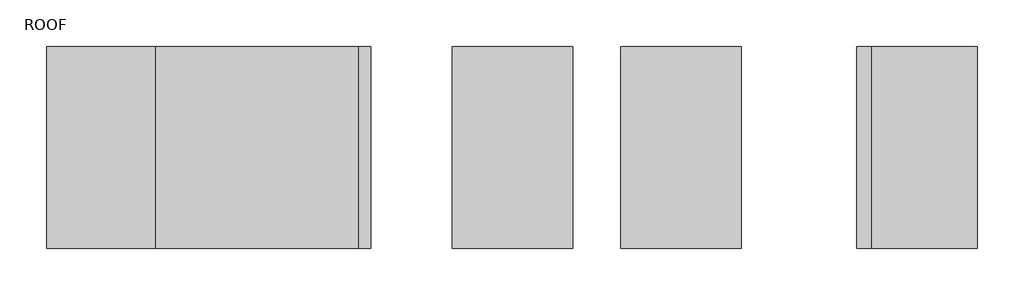
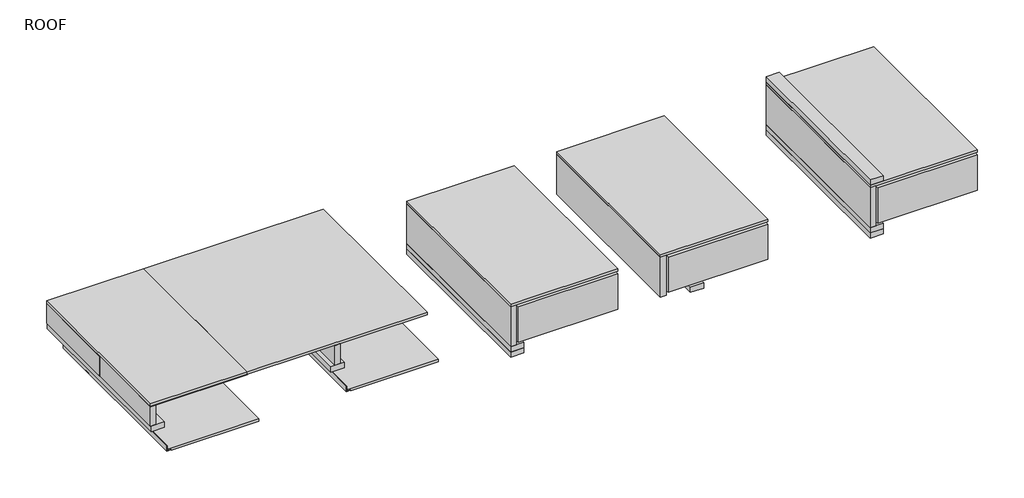
# One storey: 38 proxies.
"""IFC4 building model written with IfcOpenShell, lengths in millimetres."""

import ifcopenshell
import ifcopenshell.guid

model = None  # the IFC model being written
_history = None  # IfcOwnerHistory: only IFC2X3 demands one
_inside = {}  # id of a spatial element -> (the spatial element, [elements in it])
_under = {}  # id of a project, library or spatial element -> (it, [spatial elements below it])
_declared = {}  # id of a project -> (the project, [libraries it declares])
_typed = {}  # id of a type object -> (the type object, [elements of that type])
_made_of = {}  # id of a material, layer set ... -> (it, [elements and type objects made of it])


def new_model(schema):
    """Start an empty IFC model of exactly this schema.

    Asked for "IFC4X3", IfcOpenShell would pick the latest addendum, in which some entities
    have other attributes; the version numbers below select the first issue.
    IFC2X3 requires an IfcOwnerHistory on every rooted entity: one is made here for all.
    """
    global model, _history
    if schema == "IFC4X3":
        model = ifcopenshell.file(schema_version=(4, 3, 0, 0))
    else:
        model = ifcopenshell.file(schema=schema)
    _inside.clear()
    _under.clear()
    _declared.clear()
    _typed.clear()
    _made_of.clear()
    _history = None
    if model.schema == "IFC2X3":
        org = make("IfcOrganization", Name="unknown")
        user = make(
            "IfcPersonAndOrganization",
            ThePerson=make("IfcPerson", FamilyName="unknown"),
            TheOrganization=org,
        )
        app = make(
            "IfcApplication",
            ApplicationDeveloper=org,
            Version="unknown",
            ApplicationFullName="unknown",
            ApplicationIdentifier="unknown",
        )
        _history = make(
            "IfcOwnerHistory",
            OwningUser=user,
            OwningApplication=app,
            ChangeAction="ADDED",
            CreationDate=0,
        )
    return model


def make(cls, **values):
    """One entity of the class cls with the attributes given. An attribute that is None is left unset."""
    return model.create_entity(
        cls, **{name: value for name, value in values.items() if value is not None}
    )


def rooted(cls, **values):
    """An entity with a GlobalId (a new one), such as an element, a storey or a relation."""
    return make(cls, GlobalId=ifcopenshell.guid.new(), OwnerHistory=_history, **values)


def si_unit(unit_type, name, prefix=None):
    """IfcSIUnit, for example si_unit("LENGTHUNIT", "METRE", prefix="MILLI")."""
    return make("IfcSIUnit", UnitType=unit_type, Prefix=prefix, Name=name)


def assignment(units):
    """IfcUnitAssignment: the units of a project."""
    return None if units is None else make("IfcUnitAssignment", Units=units)


def point(xyz):
    """IfcCartesianPoint."""
    return None if xyz is None else make("IfcCartesianPoint", Coordinates=xyz)


def direction(xyz):
    """IfcDirection."""
    return None if xyz is None else make("IfcDirection", DirectionRatios=xyz)


def frame(location, z_axis=None, x_axis=None):
    """IfcAxis2Placement3D, a coordinate frame: its origin and axes. An axis left out is left unset."""
    return make(
        "IfcAxis2Placement3D",
        Location=point(location),
        Axis=direction(z_axis),
        RefDirection=direction(x_axis),
    )


def origin():
    """The frame at (0, 0, 0) with its axes left unset."""
    return frame((0.0, 0.0, 0.0))


def place(relative_to, where):
    """IfcLocalPlacement: puts the frame where relative to a parent placement (None: the world)."""
    return make(
        "IfcLocalPlacement", PlacementRelTo=relative_to, RelativePlacement=where
    )


def context(
    kind, dimensions, precision=None, world=None, true_north=None, identifier=None
):
    """IfcGeometricRepresentationContext, for example the 3D "Model" context."""
    return make(
        "IfcGeometricRepresentationContext",
        ContextIdentifier=identifier,
        ContextType=kind,
        CoordinateSpaceDimension=dimensions,
        Precision=precision,
        WorldCoordinateSystem=world,
        TrueNorth=true_north,
    )


def project(units=None, contexts=None):
    """IfcProject with its units and contexts."""
    return rooted(
        "IfcProject",
        Name="project",
        RepresentationContexts=contexts,
        UnitsInContext=assignment(units),
    )


def spatial(cls, under=None, at=None, **own):
    """A site, building, storey or space (cls), placed at a placement, below another one or the project."""
    s = rooted(cls, ObjectPlacement=at, **own)
    if under is not None:
        _under.setdefault(under.id(), (under, []))[1].append(s)
    return s


def polyline(points):
    """IfcPolyline through the points."""
    return make("IfcPolyline", Points=[point(p) for p in points])


def outline(outer, holes=None, kind="AREA"):
    """IfcArbitraryClosedProfileDef: a profile drawn as a closed curve; with holes, ...WithVoids."""
    if holes is None:
        return make("IfcArbitraryClosedProfileDef", ProfileType=kind, OuterCurve=outer)
    return make(
        "IfcArbitraryProfileDefWithVoids",
        ProfileType=kind,
        OuterCurve=outer,
        InnerCurves=holes,
    )


def extrude(swept, where, along, depth):
    """IfcExtrudedAreaSolid: the profile swept, set in the frame where, extruded along a direction by depth."""
    return make(
        "IfcExtrudedAreaSolid",
        SweptArea=swept,
        Position=where,
        ExtrudedDirection=direction(along),
        Depth=depth,
    )


def shape(context_of_items, identifier, shape_type, items):
    """IfcShapeRepresentation: the items that make up one representation, for example the "Body"."""
    return make(
        "IfcShapeRepresentation",
        ContextOfItems=context_of_items,
        RepresentationIdentifier=identifier,
        RepresentationType=shape_type,
        Items=items,
    )


def source(mapping_origin, context_of_items, identifier, shape_type, items):
    """IfcRepresentationMap: a shape defined once, which mapped items show again and again."""
    return make(
        "IfcRepresentationMap",
        MappingOrigin=mapping_origin,
        MappedRepresentation=shape(context_of_items, identifier, shape_type, items),
    )


def transform(
    local_origin,
    x_axis=None,
    y_axis=None,
    z_axis=None,
    scale=None,
    scale2=None,
    scale3=None,
    uniform=True,
):
    """IfcCartesianTransformationOperator3D, or its non-uniform kind. x_axis, y_axis, z_axis: its Axis1, 2, 3."""
    if uniform:
        return make(
            "IfcCartesianTransformationOperator3D",
            Axis1=direction(x_axis),
            Axis2=direction(y_axis),
            LocalOrigin=point(local_origin),
            Scale=scale,
            Axis3=direction(z_axis),
        )
    return make(
        "IfcCartesianTransformationOperator3DnonUniform",
        Axis1=direction(x_axis),
        Axis2=direction(y_axis),
        LocalOrigin=point(local_origin),
        Scale=scale,
        Axis3=direction(z_axis),
        Scale2=scale2,
        Scale3=scale3,
    )


def mapped(mapping_source, mapping_target):
    """IfcMappedItem: shows the shape of a source again, moved by a transform."""
    return make(
        "IfcMappedItem", MappingSource=mapping_source, MappingTarget=mapping_target
    )


def made_of(thing, what):
    """Note that an element or type object is made of a material, layer set ...; save() writes the relation."""
    if what is not None:
        _made_of.setdefault(what.id(), (what, []))[1].append(thing)
    return thing


def element(
    cls,
    number,
    at=None,
    inside=None,
    cuts=None,
    type_object=None,
    material=None,
    context=None,
    identifier="Body",
    shape_type=None,
    held_by="IfcProductDefinitionShape",
    body=None,
    shapes=None,
    **own,
):
    """One element of the class cls, such as IfcWall. Its Tag is "e" and its number.

    at: its placement. inside: the storey or other place that contains it. cuts: it is an
    opening in that element (IfcRelVoidsElement). A single representation is given by context,
    identifier, shape_type and body (its items); several are given by shapes. held_by: the class
    of the entity that holds the representations. save() writes the other relations.
    """
    e = rooted(cls, Tag="e%d" % number, ObjectPlacement=at, **own)
    if body is not None:
        shapes = [shape(context, identifier, shape_type, body)]
    if shapes is not None:
        e.Representation = make(held_by, Representations=shapes)
    if inside is not None:
        _inside.setdefault(inside.id(), (inside, []))[1].append(e)
    if cuts is not None:
        rooted(
            "IfcRelVoidsElement", RelatingBuildingElement=cuts, RelatedOpeningElement=e
        )
    if type_object is not None:
        _typed.setdefault(type_object.id(), (type_object, []))[1].append(e)
    return made_of(e, material)


def aggregate(whole, parts):
    """IfcRelAggregates: a whole, such as a stair, and the parts it consists of."""
    return rooted("IfcRelAggregates", RelatingObject=whole, RelatedObjects=parts)


def save(model, path):
    """Write the relations noted so far, then the file.

    IfcRelAggregates (storeys below a building ...), IfcRelContainedInSpatialStructure (elements
    in a storey), IfcRelDefinesByType, IfcRelAssociatesMaterial and IfcRelDeclares: one each for
    every whole, place, type object, material and project.
    """
    for whole, parts in _under.values():
        aggregate(whole, parts)
    for where, things in _inside.values():
        rooted(
            "IfcRelContainedInSpatialStructure",
            RelatedElements=things,
            RelatingStructure=where,
        )
    for kind, things in _typed.values():
        rooted("IfcRelDefinesByType", RelatedObjects=things, RelatingType=kind)
    for what, things in _made_of.values():
        rooted("IfcRelAssociatesMaterial", RelatedObjects=things, RelatingMaterial=what)
    for by, libraries in _declared.values():
        rooted("IfcRelDeclares", RelatingContext=by, RelatedDefinitions=libraries)
    model.write(path)


def generic_models_10_generic_models_1_ea081297(model_context):
    return source(origin(), model_context, "Body", "SweptSolid", [
        extrude(outline(polyline([(49758.6, 0.0), (49720.5, 0.0), (49720.5, 1219.2), (49758.6, 1219.2), (49758.6, 0.0)])), frame((0.0, 0.0, 5507.83125), z_axis=(0.0, 0.0, 1.0), x_axis=(1.0, 0.0, 0.0)), (0.0, 0.0, 1.0), 139.7),
    ])


def generic_models_109_generic_models_1_8619d77b(model_context):
    return source(origin(), model_context, "Body", "SweptSolid", [
        extrude(outline(polyline([(51003.2, 0.0), (50914.3, 0.0), (50914.3, 1219.2), (51003.2, 1219.2), (51003.2, 0.0)])), frame((0.0, 0.0, 5184.378125), z_axis=(0.0, 0.0, 1.0), x_axis=(1.0, 0.0, 0.0)), (0.0, 0.0, 1.0), 38.1),
    ])


def generic_models_110_generic_models_1_6bdce9b6(model_context):
    return source(origin(), model_context, "Body", "SweptSolid", [
        extrude(outline(polyline([(51642.1451407, 1219.2), (51642.1451407, 0.0), (50914.3, 0.0), (50914.3, 1219.2), (51642.1451407, 1219.2)])), frame((0.0, 0.0, 5508.228125), z_axis=(0.0, 0.0, 1.0), x_axis=(1.0, 0.0, 0.0)), (0.0, 0.0, 1.0), 19.05),
    ])


def generic_models_112_generic_models_65_d168d7b0(model_context):
    return source(origin(), model_context, "Body", "SweptSolid", [
        extrude(outline(polyline([(50952.4, 592.1375), (50952.4, 630.2375), (51642.1451407, 630.2375), (51642.1451407, 592.1375), (50952.4, 592.1375)])), frame((0.0, 0.0, 5222.478125), z_axis=(0.0, 0.0, 1.0), x_axis=(1.0, 0.0, 0.0)), (0.0, 0.0, 1.0), 285.75),
    ])


def generic_models_113_generic_models_1_101608ab(model_context):
    return source(origin(), model_context, "Body", "SweptSolid", [
        extrude(outline(polyline([(52171.6, 0.0), (52133.5, 0.0), (52133.5, 1219.2), (52171.6, 1219.2), (52171.6, 0.0)])), frame((0.0, 0.0, 5222.478125), z_axis=(0.0, 0.0, 1.0), x_axis=(1.0, 0.0, 0.0)), (0.0, 0.0, 1.0), 285.75),
    ])


def generic_models_114_generic_models_1_a6fb1c2c(model_context):
    return source(origin(), model_context, "Body", "SweptSolid", [
        extrude(outline(polyline([(51642.1451407, 1219.2), (51642.1451407, 0.0), (50965.9242022, 0.0), (50965.9242022, 1219.2), (51642.1451407, 1219.2)])), frame((0.0, 0.0, 5237.6235034), z_axis=(0.0, 0.0, 1.0), x_axis=(1.0, 0.0, 0.0)), (0.0, 0.0, 1.0), 254.0),
    ])


def generic_models_12_generic_models_46_b8a9a4e8(model_context):
    return source(origin(), model_context, "Body", "SweptSolid", [
        extrude(outline(polyline([(49757.8505137, 0.0), (49721.1284797, 0.0), (49721.1284797, 1219.2), (49757.8505137, 1219.2), (49757.8505137, 0.0)])), frame((0.0, 0.0, 5505.7509163), z_axis=(0.0, 0.0, 1.0), x_axis=(1.0, 0.0, 0.0)), (0.0, 0.0, 1.0), 1.5875),
    ])


def generic_models_13_generic_models_65_9e643fb9(model_context):
    return source(origin(), model_context, "Body", "SweptSolid", [
        extrude(outline(polyline([(49128.3625, 592.1375), (49128.3625, 630.2375), (50347.5625, 630.2375), (50347.5625, 592.1375), (49128.3625, 592.1375)])), frame((0.0, 0.0, 5507.83125), z_axis=(0.0, 0.0, 1.0), x_axis=(1.0, 0.0, 0.0)), (0.0, 0.0, 1.0), 139.7),
    ])


def generic_models_14_generic_models_1_e8c90d4c(model_context):
    return source(origin(), model_context, "Body", "SweptSolid", [
        extrude(outline(polyline([(2277.1204978, 49799.875), (2239.0204978, 49799.875), (2239.0204978, 49825.275), (2240.6079978, 49825.275), (2240.6079978, 49801.4625), (2277.1204978, 49801.4625), (2277.1204978, 49799.875)])), frame((0.0, 0.0, 0.0), z_axis=(0.0, 1.0, 0.0), x_axis=(0.0, 0.0, 1.0)), (0.0, 0.0, 1.0), 1219.2),
    ])


def generic_models_22_generic_models_1_e5767157(model_context):
    return source(origin(), model_context, "Body", "SweptSolid", [
        extrude(outline(polyline([(2409.6091, 49800.66875), (2409.6091, 49799.875), (2407.0592364, 49799.875), (2405.4618473, 49749.075), (2404.6631527, 49749.075), (2403.0657636, 49799.875), (2400.5159, 49799.875), (2400.5159, 49800.66875), (2409.6091, 49800.66875)])), frame((0.0, 565.15, 0.0), z_axis=(0.0, 1.0, 0.0), x_axis=(0.0, 0.0, 1.0)), (0.0, 0.0, 1.0), 12.7),
    ])


def generic_models_226_generic_models_1_7dc37832(model_context):
    return source(origin(), model_context, "Body", "SweptSolid", [
        extrude(outline(polyline([(5263.35625, 49733.4159), (5263.35625, 49742.5091), (5264.15, 49742.5091), (5264.15, 49739.9592364), (5314.95, 49738.3618473), (5314.95, 49737.5631527), (5264.15, 49735.9657636), (5264.15, 49733.4159), (5263.35625, 49733.4159)])), frame((0.0, 565.15, 0.0), z_axis=(0.0, 1.0, 0.0), x_axis=(0.0, 0.0, 1.0)), (0.0, 0.0, 1.0), 12.7),
    ])


def generic_models_202_generic_models_1_0ad20a8b(model_context):
    return source(origin(), model_context, "Body", "SweptSolid", [
        extrude(outline(polyline([(2253.330428, 49813.3451407), (2242.217928, 49813.3451407), (2242.217928, 49826.0451407), (2234.280428, 49828.9341545), (2234.280428, 50422.9451407), (2253.330428, 50422.9451407), (2253.330428, 49813.3451407)])), frame((0.0, 0.0, 0.0), z_axis=(0.0, 1.0, 0.0), x_axis=(0.0, 0.0, 1.0)), (0.0, 0.0, 1.0), 1219.2),
    ])


def generic_models_233_generic_models_1_ae5bae41(model_context):
    return source(origin(), model_context, "Body", "SweptSolid", [
        extrude(outline(polyline([(48564.8, 0.0), (48475.9, 0.0), (48475.9, 1219.2), (48564.8, 1219.2), (48564.8, 0.0)])), frame((0.0, 0.0, 5467.35), z_axis=(0.0, 0.0, 1.0), x_axis=(1.0, 0.0, 0.0)), (0.0, 0.0, 1.0), 38.1),
    ])


def generic_models_236_generic_models_1_f8917e71(model_context):
    return source(origin(), model_context, "Body", "SweptSolid", [
        extrude(outline(polyline([(48507.65, 0.0), (48469.55, 0.0), (48469.55, 1219.2), (48507.65, 1219.2), (48507.65, 0.0)])), frame((0.0, 0.0, 5507.83125), z_axis=(0.0, 0.0, 1.0), x_axis=(1.0, 0.0, 0.0)), (0.0, 0.0, 1.0), 139.7),
    ])


def generic_models_237_generic_models_65_1df05f16(model_context):
    return source(origin(), model_context, "Body", "SweptSolid", [
        extrude(outline(polyline([(48469.55, 592.1375), (48469.55, 630.2375), (49128.3625, 630.2375), (49128.3625, 592.1375), (48469.55, 592.1375)])), frame((0.0, 0.0, 5507.83125), z_axis=(0.0, 0.0, 1.0), x_axis=(1.0, 0.0, 0.0)), (0.0, 0.0, 1.0), 139.7),
    ])


def generic_models_239_generic_models_46_95e6735a(model_context):
    return source(origin(), model_context, "Body", "SweptSolid", [
        extrude(outline(polyline([(50347.5625, 0.0), (49691.4320511, 0.0), (49691.4320511, 1219.2), (50347.5625, 1219.2), (50347.5625, 0.0)])), frame((0.0, 0.0, 5505.7509163), z_axis=(0.0, 0.0, 1.0), x_axis=(1.0, 0.0, 0.0)), (0.0, 0.0, 1.0), 1.5875),
    ])


def generic_models_240_generic_models_1_611786cf(model_context):
    return source(origin(), model_context, "Body", "SweptSolid", [
        extrude(outline(polyline([(49128.3625, 1219.2), (49128.3625, 0.0), (48469.55, 0.0), (48469.55, 1219.2), (49128.3625, 1219.2)])), frame((0.0, 0.0, 5649.9125), z_axis=(0.0, 0.0, 1.0), x_axis=(1.0, 0.0, 0.0)), (0.0, 0.0, 1.0), 19.05),
    ])


def generic_models_29_generic_models_1_59087225(model_context):
    return source(origin(), model_context, "Body", "SweptSolid", [
        extrude(outline(polyline([(50347.5625, 1219.2), (50347.5625, 0.0), (49128.3625, 0.0), (49128.3625, 1219.2), (50347.5625, 1219.2)])), frame((0.0, 0.0, 5647.53125), z_axis=(0.0, 0.0, 1.0), x_axis=(1.0, 0.0, 0.0)), (0.0, 0.0, 1.0), 19.05),
    ])


def generic_models_37_generic_models_1_916dd7c6(model_context):
    return source(origin(), model_context, "Body", "SweptSolid", [
        extrude(outline(polyline([(2409.6091, 49675.25625), (2400.5159, 49675.25625), (2400.5159, 49676.05), (2403.0657636, 49676.05), (2404.6631527, 49726.85), (2405.4618473, 49726.85), (2407.0592364, 49676.05), (2409.6091, 49676.05), (2409.6091, 49675.25625)])), frame((0.0, 565.15, 0.0), z_axis=(0.0, 1.0, 0.0), x_axis=(0.0, 0.0, 1.0)), (0.0, 0.0, 1.0), 12.7),
    ])


def generic_models_103_generic_models_1_250a6a11(model_context):
    return source(origin(), model_context, "Body", "SweptSolid", [
        extrude(outline(polyline([(49784.0, 0.0), (49695.1, 0.0), (49695.1, 1219.2), (49784.0, 1219.2), (49784.0, 0.0)])), frame((0.0, 0.0, 5264.15), z_axis=(0.0, 0.0, 1.0), x_axis=(1.0, 0.0, 0.0)), (0.0, 0.0, 1.0), 38.1),
    ])


def generic_models_71_generic_models_1_508a995f(model_context):
    return source(origin(), model_context, "Body", "SweptSolid", [
        extrude(outline(polyline([(50952.4, 0.0), (50914.3, 0.0), (50914.3, 1219.2), (50952.4, 1219.2), (50952.4, 0.0)])), frame((0.0, 0.0, 5222.478125), z_axis=(0.0, 0.0, 1.0), x_axis=(1.0, 0.0, 0.0)), (0.0, 0.0, 1.0), 285.75),
    ])


def generic_models_87_generic_models_1_55a64953(model_context):
    return source(origin(), model_context, "Body", "SweptSolid", [
        extrude(outline(polyline([(51968.4, 0.0), (51930.3, 0.0), (51930.3, 1219.2), (51968.4, 1219.2), (51968.4, 0.0)])), frame((0.0, 0.0, 5222.478125), z_axis=(0.0, 0.0, 1.0), x_axis=(1.0, 0.0, 0.0)), (0.0, 0.0, 1.0), 285.75),
    ])


model = new_model("IFC4")

# Units and contexts
model_context = context("Model", 3, world=origin())
ifc_project = project(units=[si_unit("LENGTHUNIT", "METRE", prefix="MILLI")], contexts=[model_context])

# Site, building, storey
site = spatial("IfcSite", under=ifc_project)
building = spatial("IfcBuilding", under=site)
storey = spatial("IfcBuildingStorey", under=building, Name="ROOF", Elevation=5130.8)

# Proxies
placement = place(None, origin())
generic_models_10_generic_models_1_shape = generic_models_10_generic_models_1_ea081297(model_context)
element("IfcBuildingElementProxy", 1, Name="Generic Models 10 : Generic Models 1", ObjectType="Generic Models 10 : Generic Models 1", at=placement, inside=storey, context=model_context, shape_type="MappedRepresentation", body=[
    mapped(generic_models_10_generic_models_1_shape, transform((0.0, 0.0, 0.0), x_axis=(1.0, 0.0, 0.0), y_axis=(0.0, 1.0, 0.0), z_axis=(0.0, 0.0, 1.0))),
])
generic_models_109_generic_models_1_shape = generic_models_109_generic_models_1_8619d77b(model_context)
element("IfcBuildingElementProxy", 2, Name="Generic Models 109 : Generic Models 1", ObjectType="Generic Models 109 : Generic Models 1", at=placement, inside=storey, context=model_context, shape_type="MappedRepresentation", body=[
    mapped(generic_models_109_generic_models_1_shape, transform((2438.4, 0.0, 0.0), x_axis=(1.0, 0.0, 0.0), y_axis=(0.0, 1.0, 0.0), z_axis=(0.0, 0.0, 1.0))),
])
generic_models_110_generic_models_1_shape = generic_models_110_generic_models_1_6bdce9b6(model_context)
element("IfcBuildingElementProxy", 3, Name="Generic Models 110 : Generic Models 1", ObjectType="Generic Models 110 : Generic Models 1", at=placement, inside=storey, context=model_context, shape_type="MappedRepresentation", body=[
    mapped(generic_models_110_generic_models_1_shape, transform((2438.4, 0.0, 0.0), x_axis=(1.0, 0.0, 0.0), y_axis=(0.0, 1.0, 0.0), z_axis=(0.0, 0.0, 1.0))),
])
element("IfcBuildingElementProxy", 4, Name="Generic Models 111 : Generic Models 1", ObjectType="Generic Models 111 : Generic Models 1", at=placement, inside=storey, context=model_context, shape_type="MappedRepresentation", body=[
    mapped(generic_models_109_generic_models_1_shape, transform((2438.4, 0.0, -38.1), x_axis=(1.0, 0.0, 0.0), y_axis=(0.0, 1.0, 0.0), z_axis=(0.0, 0.0, 1.0))),
])
generic_models_112_generic_models_65_shape = generic_models_112_generic_models_65_d168d7b0(model_context)
element("IfcBuildingElementProxy", 5, Name="Generic Models 112 : Generic Models 65", ObjectType="Generic Models 112 : Generic Models 65", at=placement, inside=storey, context=model_context, shape_type="MappedRepresentation", body=[
    mapped(generic_models_112_generic_models_65_shape, transform((2438.4, 0.0, 0.0), x_axis=(1.0, 0.0, 0.0), y_axis=(0.0, 1.0, 0.0), z_axis=(0.0, 0.0, 1.0))),
])
generic_models_113_generic_models_1_shape = generic_models_113_generic_models_1_101608ab(model_context)
element("IfcBuildingElementProxy", 6, Name="Generic Models 113 : Generic Models 1", ObjectType="Generic Models 113 : Generic Models 1", at=placement, inside=storey, context=model_context, shape_type="MappedRepresentation", body=[
    mapped(generic_models_113_generic_models_1_shape, transform((1219.2, 0.0, 0.0), x_axis=(1.0, 0.0, 0.0), y_axis=(0.0, 1.0, 0.0), z_axis=(0.0, 0.0, 1.0))),
])
generic_models_114_generic_models_1_shape = generic_models_114_generic_models_1_a6fb1c2c(model_context)
element("IfcBuildingElementProxy", 7, Name="Generic Models 114 : Generic Models 1", ObjectType="Generic Models 114 : Generic Models 1", at=placement, inside=storey, context=model_context, shape_type="MappedRepresentation", body=[
    mapped(generic_models_114_generic_models_1_shape, transform((2438.4, 0.0, 0.0), x_axis=(1.0, 0.0, 0.0), y_axis=(0.0, 1.0, 0.0), z_axis=(0.0, 0.0, 1.0))),
])
element("IfcBuildingElementProxy", 8, Name="Generic Models 115 : Generic Models 1", ObjectType="Generic Models 115 : Generic Models 1", at=placement, inside=storey, context=model_context, shape_type="MappedRepresentation", body=[
    mapped(generic_models_109_generic_models_1_shape, transform((2438.4, 0.0, 342.9), x_axis=(1.0, 0.0, 0.0), y_axis=(0.0, 1.0, 0.0), z_axis=(0.0, 0.0, 1.0))),
])
generic_models_12_generic_models_46_shape = generic_models_12_generic_models_46_b8a9a4e8(model_context)
element("IfcBuildingElementProxy", 9, Name="Generic Models 12 : Generic Models 46", ObjectType="Generic Models 12 : Generic Models 46", at=placement, inside=storey, context=model_context, shape_type="MappedRepresentation", body=[
    mapped(generic_models_12_generic_models_46_shape, transform((0.0, 0.0, 0.0), x_axis=(1.0, 0.0, 0.0), y_axis=(0.0, 1.0, 0.0), z_axis=(0.0, 0.0, 1.0))),
])
generic_models_13_generic_models_65_shape = generic_models_13_generic_models_65_9e643fb9(model_context)
element("IfcBuildingElementProxy", 10, Name="Generic Models 13 : Generic Models 65", ObjectType="Generic Models 13 : Generic Models 65", at=placement, inside=storey, context=model_context, shape_type="MappedRepresentation", body=[
    mapped(generic_models_13_generic_models_65_shape, transform((0.0, 0.0, 0.0), x_axis=(1.0, 0.0, 0.0), y_axis=(0.0, 1.0, 0.0), z_axis=(0.0, 0.0, 1.0))),
])
generic_models_14_generic_models_1_shape = generic_models_14_generic_models_1_e8c90d4c(model_context)
element("IfcBuildingElementProxy", 11, Name="Generic Models 14 : Generic Models 1", ObjectType="Generic Models 14 : Generic Models 1", at=placement, inside=storey, context=model_context, shape_type="MappedRepresentation", body=[
    mapped(generic_models_14_generic_models_1_shape, transform((0.0, 0.0, 3050.778125), x_axis=(1.0, 0.0, 0.0), y_axis=(0.0, 1.0, 0.0), z_axis=(0.0, 0.0, 1.0))),
])
generic_models_22_generic_models_1_shape = generic_models_22_generic_models_1_e5767157(model_context)
element("IfcBuildingElementProxy", 12, Name="Generic Models 22 : Generic Models 1", ObjectType="Generic Models 22 : Generic Models 1", at=placement, inside=storey, context=model_context, shape_type="MappedRepresentation", body=[
    mapped(generic_models_22_generic_models_1_shape, transform((0.0, 0.0, 3081.3375), x_axis=(1.0, 0.0, 0.0), y_axis=(0.0, 1.0, 0.0), z_axis=(0.0, 0.0, 1.0))),
])
element("IfcBuildingElementProxy", 13, Name="Generic Models 224 : Generic Models 1", ObjectType="Generic Models 224 : Generic Models 1", at=placement, inside=storey, context=model_context, shape_type="MappedRepresentation", body=[
    mapped(generic_models_14_generic_models_1_shape, transform((-1217.6125, 0.0, 3050.778125), x_axis=(1.0, 0.0, 0.0), y_axis=(0.0, 1.0, 0.0), z_axis=(0.0, 0.0, 1.0))),
])
element("IfcBuildingElementProxy", 14, Name="Generic Models 225 : Generic Models 1", ObjectType="Generic Models 225 : Generic Models 1", at=placement, inside=storey, context=model_context, shape_type="MappedRepresentation", body=[
    mapped(generic_models_22_generic_models_1_shape, transform((-1219.2, 0.0, 3081.3375), x_axis=(1.0, 0.0, 0.0), y_axis=(0.0, 1.0, 0.0), z_axis=(0.0, 0.0, 1.0))),
])
generic_models_226_generic_models_1_shape = generic_models_226_generic_models_1_7dc37832(model_context)
element("IfcBuildingElementProxy", 15, Name="Generic Models 226 : Generic Models 1", ObjectType="Generic Models 226 : Generic Models 1", at=placement, inside=storey, context=model_context, shape_type="MappedRepresentation", body=[
    mapped(generic_models_226_generic_models_1_shape, transform((-1219.2, 0.0, 203.2), x_axis=(1.0, 0.0, 0.0), y_axis=(0.0, 1.0, 0.0), z_axis=(0.0, 0.0, 1.0))),
])
generic_models_202_generic_models_1_shape = generic_models_202_generic_models_1_0ad20a8b(model_context)
element("IfcBuildingElementProxy", 16, Name="Generic Models 231 : Generic Models 1", ObjectType="Generic Models 231 : Generic Models 1", at=placement, inside=storey, context=model_context, shape_type="MappedRepresentation", body=[
    mapped(generic_models_202_generic_models_1_shape, transform((-1217.6125, 0.0, 3050.778125), x_axis=(1.0, 0.0, 0.0), y_axis=(0.0, 1.0, 0.0), z_axis=(0.0, 0.0, 1.0))),
])
generic_models_233_generic_models_1_shape = generic_models_233_generic_models_1_ae5bae41(model_context)
element("IfcBuildingElementProxy", 17, Name="Generic Models 233 : Generic Models 1", ObjectType="Generic Models 233 : Generic Models 1", at=placement, inside=storey, context=model_context, shape_type="MappedRepresentation", body=[
    mapped(generic_models_233_generic_models_1_shape, transform((0.0, 0.0, 0.0), x_axis=(1.0, 0.0, 0.0), y_axis=(0.0, 1.0, 0.0), z_axis=(0.0, 0.0, 1.0))),
])
generic_models_236_generic_models_1_shape = generic_models_236_generic_models_1_f8917e71(model_context)
element("IfcBuildingElementProxy", 18, Name="Generic Models 236 : Generic Models 1", ObjectType="Generic Models 236 : Generic Models 1", at=placement, inside=storey, context=model_context, shape_type="MappedRepresentation", body=[
    mapped(generic_models_236_generic_models_1_shape, transform((0.0, 0.0, 0.0), x_axis=(1.0, 0.0, 0.0), y_axis=(0.0, 1.0, 0.0), z_axis=(0.0, 0.0, 1.0))),
])
generic_models_237_generic_models_65_shape = generic_models_237_generic_models_65_1df05f16(model_context)
element("IfcBuildingElementProxy", 19, Name="Generic Models 237 : Generic Models 65", ObjectType="Generic Models 237 : Generic Models 65", at=placement, inside=storey, context=model_context, shape_type="MappedRepresentation", body=[
    mapped(generic_models_237_generic_models_65_shape, transform((0.0, 0.0, 0.0), x_axis=(1.0, 0.0, 0.0), y_axis=(0.0, 1.0, 0.0), z_axis=(0.0, 0.0, 1.0))),
])
generic_models_239_generic_models_46_shape = generic_models_239_generic_models_46_95e6735a(model_context)
element("IfcBuildingElementProxy", 20, Name="Generic Models 239 : Generic Models 46", ObjectType="Generic Models 239 : Generic Models 46", at=placement, inside=storey, context=model_context, shape_type="MappedRepresentation", body=[
    mapped(generic_models_239_generic_models_46_shape, transform((-1219.2, 0.0, 142.08125), x_axis=(1.0, 0.0, 0.0), y_axis=(0.0, 1.0, 0.0), z_axis=(0.0, 0.0, 1.0))),
])
generic_models_240_generic_models_1_shape = generic_models_240_generic_models_1_611786cf(model_context)
element("IfcBuildingElementProxy", 21, Name="Generic Models 240 : Generic Models 1", ObjectType="Generic Models 240 : Generic Models 1", at=placement, inside=storey, context=model_context, shape_type="MappedRepresentation", body=[
    mapped(generic_models_240_generic_models_1_shape, transform((0.0, 0.0, 0.0), x_axis=(1.0, 0.0, 0.0), y_axis=(0.0, 1.0, 0.0), z_axis=(0.0, 0.0, 1.0))),
])
element("IfcBuildingElementProxy", 22, Name="Generic Models 25 : Generic Models 46", ObjectType="Generic Models 25 : Generic Models 46", at=placement, inside=storey, context=model_context, shape_type="MappedRepresentation", body=[
    mapped(generic_models_12_generic_models_46_shape, transform((0.0, 0.0, 142.08125), x_axis=(1.0, 0.0, 0.0), y_axis=(0.0, 1.0, 0.0), z_axis=(0.0, 0.0, 1.0))),
])
generic_models_29_generic_models_1_shape = generic_models_29_generic_models_1_59087225(model_context)
element("IfcBuildingElementProxy", 23, Name="Generic Models 29 : Generic Models 1", ObjectType="Generic Models 29 : Generic Models 1", at=placement, inside=storey, context=model_context, shape_type="MappedRepresentation", body=[
    mapped(generic_models_29_generic_models_1_shape, transform((0.0, 0.0, 2.38125), x_axis=(1.0, 0.0, 0.0), y_axis=(0.0, 1.0, 0.0), z_axis=(0.0, 0.0, 1.0))),
])
element("IfcBuildingElementProxy", 24, Name="Generic Models 39 : Generic Models 1", ObjectType="Generic Models 39 : Generic Models 1", at=placement, inside=storey, context=model_context, shape_type="MappedRepresentation", body=[
    mapped(generic_models_226_generic_models_1_shape, transform((0.0, 0.0, 203.2), x_axis=(1.0, 0.0, 0.0), y_axis=(0.0, 1.0, 0.0), z_axis=(0.0, 0.0, 1.0))),
])
generic_models_37_generic_models_1_shape = generic_models_37_generic_models_1_916dd7c6(model_context)
element("IfcBuildingElementProxy", 25, Name="Generic Models 47 : Generic Models 1", ObjectType="Generic Models 47 : Generic Models 1", at=placement, inside=storey, context=model_context, shape_type="MappedRepresentation", body=[
    mapped(generic_models_37_generic_models_1_shape, transform((3.175, 0.0, 3081.3375), x_axis=(1.0, 0.0, 0.0), y_axis=(0.0, 1.0, 0.0), z_axis=(0.0, 0.0, 1.0))),
])
element("IfcBuildingElementProxy", 26, Name="Generic Models 49 : Generic Models 1", ObjectType="Generic Models 49 : Generic Models 1", at=placement, inside=storey, context=model_context, shape_type="MappedRepresentation", body=[
    mapped(generic_models_202_generic_models_1_shape, transform((0.0, 0.0, 3050.778125), x_axis=(1.0, 0.0, 0.0), y_axis=(0.0, 1.0, 0.0), z_axis=(0.0, 0.0, 1.0))),
])
element("IfcBuildingElementProxy", 27, Name="Generic Models 59 : Generic Models 65", ObjectType="Generic Models 59 : Generic Models 65", at=placement, inside=storey, context=model_context, shape_type="MappedRepresentation", body=[
    mapped(generic_models_112_generic_models_65_shape, transform((0.0, 0.0, 0.0), x_axis=(1.0, 0.0, 0.0), y_axis=(0.0, 1.0, 0.0), z_axis=(0.0, 0.0, 1.0))),
])
generic_models_103_generic_models_1_shape = generic_models_103_generic_models_1_250a6a11(model_context)
element("IfcBuildingElementProxy", 28, Name="Generic Models 6 : Generic Models 1", ObjectType="Generic Models 6 : Generic Models 1", at=placement, inside=storey, context=model_context, shape_type="MappedRepresentation", body=[
    mapped(generic_models_103_generic_models_1_shape, transform((0.0, 0.0, 203.2), x_axis=(1.0, 0.0, 0.0), y_axis=(0.0, 1.0, 0.0), z_axis=(0.0, 0.0, 1.0))),
])
element("IfcBuildingElementProxy", 29, Name="Generic Models 64 : Generic Models 1", ObjectType="Generic Models 64 : Generic Models 1", at=placement, inside=storey, context=model_context, shape_type="MappedRepresentation", body=[
    mapped(generic_models_109_generic_models_1_shape, transform((0.0, 0.0, 0.0), x_axis=(1.0, 0.0, 0.0), y_axis=(0.0, 1.0, 0.0), z_axis=(0.0, 0.0, 1.0))),
])
element("IfcBuildingElementProxy", 30, Name="Generic Models 66 : Generic Models 1", ObjectType="Generic Models 66 : Generic Models 1", at=placement, inside=storey, context=model_context, shape_type="MappedRepresentation", body=[
    mapped(generic_models_110_generic_models_1_shape, transform((0.0, 0.0, 0.0), x_axis=(1.0, 0.0, 0.0), y_axis=(0.0, 1.0, 0.0), z_axis=(0.0, 0.0, 1.0))),
])
element("IfcBuildingElementProxy", 31, Name="Generic Models 70 : Generic Models 1", ObjectType="Generic Models 70 : Generic Models 1", at=placement, inside=storey, context=model_context, shape_type="MappedRepresentation", body=[
    mapped(generic_models_109_generic_models_1_shape, transform((0.0, 0.0, -38.1), x_axis=(1.0, 0.0, 0.0), y_axis=(0.0, 1.0, 0.0), z_axis=(0.0, 0.0, 1.0))),
])
generic_models_71_generic_models_1_shape = generic_models_71_generic_models_1_508a995f(model_context)
element("IfcBuildingElementProxy", 32, Name="Generic Models 71 : Generic Models 1", ObjectType="Generic Models 71 : Generic Models 1", at=placement, inside=storey, context=model_context, shape_type="MappedRepresentation", body=[
    mapped(generic_models_71_generic_models_1_shape, transform((0.0, 0.0, 0.0), x_axis=(1.0, 0.0, 0.0), y_axis=(0.0, 1.0, 0.0), z_axis=(0.0, 0.0, 1.0))),
])
element("IfcBuildingElementProxy", 33, Name="Generic Models 72 : Generic Models 1", ObjectType="Generic Models 72 : Generic Models 1", at=placement, inside=storey, context=model_context, shape_type="MappedRepresentation", body=[
    mapped(generic_models_114_generic_models_1_shape, transform((0.0, 0.0, 0.0), x_axis=(1.0, 0.0, 0.0), y_axis=(0.0, 1.0, 0.0), z_axis=(0.0, 0.0, 1.0))),
])
element("IfcBuildingElementProxy", 34, Name="Generic Models 81 : Generic Models 1", ObjectType="Generic Models 81 : Generic Models 1", at=placement, inside=storey, context=model_context, shape_type="MappedRepresentation", body=[
    mapped(generic_models_109_generic_models_1_shape, transform((1219.2, 0.0, 0.0), x_axis=(1.0, 0.0, 0.0), y_axis=(0.0, 1.0, 0.0), z_axis=(0.0, 0.0, 1.0))),
])
element("IfcBuildingElementProxy", 35, Name="Generic Models 82 : Generic Models 1", ObjectType="Generic Models 82 : Generic Models 1", at=placement, inside=storey, context=model_context, shape_type="MappedRepresentation", body=[
    mapped(generic_models_110_generic_models_1_shape, transform((1016.0, 0.0, 0.0), x_axis=(1.0, 0.0, 0.0), y_axis=(0.0, 1.0, 0.0), z_axis=(0.0, 0.0, 1.0))),
])
element("IfcBuildingElementProxy", 36, Name="Generic Models 86 : Generic Models 65", ObjectType="Generic Models 86 : Generic Models 65", at=placement, inside=storey, context=model_context, shape_type="MappedRepresentation", body=[
    mapped(generic_models_112_generic_models_65_shape, transform((1016.0, 0.0, 0.0), x_axis=(1.0, 0.0, 0.0), y_axis=(0.0, 1.0, 0.0), z_axis=(0.0, 0.0, 1.0))),
])
generic_models_87_generic_models_1_shape = generic_models_87_generic_models_1_55a64953(model_context)
element("IfcBuildingElementProxy", 37, Name="Generic Models 87 : Generic Models 1", ObjectType="Generic Models 87 : Generic Models 1", at=placement, inside=storey, context=model_context, shape_type="MappedRepresentation", body=[
    mapped(generic_models_87_generic_models_1_shape, transform((0.0, 0.0, 0.0), x_axis=(1.0, 0.0, 0.0), y_axis=(0.0, 1.0, 0.0), z_axis=(0.0, 0.0, 1.0))),
])
element("IfcBuildingElementProxy", 38, Name="Generic Models 88 : Generic Models 1", ObjectType="Generic Models 88 : Generic Models 1", at=placement, inside=storey, context=model_context, shape_type="MappedRepresentation", body=[
    mapped(generic_models_114_generic_models_1_shape, transform((1016.0, 0.0, 0.0), x_axis=(1.0, 0.0, 0.0), y_axis=(0.0, 1.0, 0.0), z_axis=(0.0, 0.0, 1.0))),
])

save(model, "model.ifc")

# Revit data of these elements
# Project information
#   Project Issue Date = "06/12/2018"
#   Project Status = "Project Status"
#   Client Name = "Owner"
#   Project Address = "5253 KING JAMES WAY, FITCHBURG, WI"
#   Project Name = "FORAGE KOMBUCHA"
#   Project Number = "Project Number"
# Grids (mm)
#   "B": line (-20559.366, -20036.147) -> (-20559.366, -4657.508)
#   "C": line (-23277.166, -20036.147) -> (-23277.166, -4657.508)
#   "D": line (-25994.966, -20036.147) -> (-25994.966, -4657.508)
# Element 1 (IfcBuildingElementProxy, "Generic Models 10 : Generic Models 1")
#   Phase Created = _ZAVE
#   Materials on its faces: "2X BLOCKING - LOCATED AT GRAB BARS, WALL HUNG CABINETS, ETC.)"
# Element 2 (IfcBuildingElementProxy, "Generic Models 109 : Generic Models 1")
#   Phase Created = _ZAVE
#   Materials on its faces: "DOUBLE 2X WOOD TOP PLATE"
# Element 3 (IfcBuildingElementProxy, "Generic Models 110 : Generic Models 1")
#   Phase Created = _ZAVE
#   Materials on its faces: "3/4\" CDX PLYWOOD"
# Element 4 (IfcBuildingElementProxy, "Generic Models 111 : Generic Models 1")
#   Phase Created = _ZAVE
#   Materials on its faces: "DOUBLE 2X WOOD TOP PLATE"
# Element 5 (IfcBuildingElementProxy, "Generic Models 112 : Generic Models 65")
#   Phase Created = _ZAVE
#   Materials on its faces: "WOOD JOIST AS SPECIFIED"
# Element 6 (IfcBuildingElementProxy, "Generic Models 113 : Generic Models 1")
#   Phase Created = _ZAVE
#   Materials on its faces: "RIM BOARD - SIZE TO MATCH JOIST DEPTH"
# Element 7 (IfcBuildingElementProxy, "Generic Models 114 : Generic Models 1")
#   Phase Created = _ZAVE
#   Materials on its faces: "SOUND BATT. INSULATION"
# Element 8 (IfcBuildingElementProxy, "Generic Models 115 : Generic Models 1")
#   Phase Created = _ZAVE
#   Materials on its faces: "DOUBLE 2X WOOD TOP PLATE"
# Element 9 (IfcBuildingElementProxy, "Generic Models 12 : Generic Models 46")
#   Phase Created = _ZAVE
#   Materials on its faces: "SET IN BED OF SEALANT"
# Element 10 (IfcBuildingElementProxy, "Generic Models 13 : Generic Models 65")
#   Phase Created = _ZAVE
#   Materials on its faces: "WOOD JOIST AS SPECIFIED"
# Element 11 (IfcBuildingElementProxy, "Generic Models 14 : Generic Models 1")
#   Phase Created = _ZAVE
#   Materials on its faces: "CEILING TRACK AS SCHEDULED"
# Element 12 (IfcBuildingElementProxy, "Generic Models 22 : Generic Models 1")
#   Phase Created = _ZAVE
#   Materials on its faces: "ATTACH GYPSUM BOARD TO STUDS AND NOT TO TOP TRACK"
# Element 13 (IfcBuildingElementProxy, "Generic Models 224 : Generic Models 1")
#   Phase Created = _ZAVE
#   Materials on its faces: "CEILING TRACK AS SCHEDULED"
# Element 14 (IfcBuildingElementProxy, "Generic Models 225 : Generic Models 1")
#   Phase Created = _ZAVE
#   Materials on its faces: "ATTACH GYPSUM BOARD TO STUDS AND NOT TO TOP TRACK"
# Element 15 (IfcBuildingElementProxy, "Generic Models 226 : Generic Models 1")
#   Phase Created = _ZAVE
#   Materials on its faces: "METAL RUNNER CHANNEL; FASTEN @ 24\" O.C."
# Element 16 (IfcBuildingElementProxy, "Generic Models 231 : Generic Models 1")
#   Phase Created = _ZAVE
#   Materials on its faces: "CEILING AS SCHEDULED"
# Element 17 (IfcBuildingElementProxy, "Generic Models 233 : Generic Models 1")
#   Phase Created = _ZAVE
#   Materials on its faces: "2X WOOD HEADER ATTACHED TO STEEL PURLIN"
# Element 18 (IfcBuildingElementProxy, "Generic Models 236 : Generic Models 1")
#   Phase Created = _ZAVE
#   Materials on its faces: "EXISTING RIM BOARD OR JOIST"
# Element 19 (IfcBuildingElementProxy, "Generic Models 237 : Generic Models 65")
#   Phase Created = _ZAVE
#   Materials on its faces: "WOOD JOIST AS SPECIFIED"
# Element 20 (IfcBuildingElementProxy, "Generic Models 239 : Generic Models 46")
#   Phase Created = _ZAVE
#   Materials on its faces: "SET IN BED OF SEALANT"
# Element 21 (IfcBuildingElementProxy, "Generic Models 240 : Generic Models 1")
#   Phase Created = _ZAVE
#   Materials on its faces: "EXISTING SUBSTRATE"
# Element 22 (IfcBuildingElementProxy, "Generic Models 25 : Generic Models 46")
#   Phase Created = _ZAVE
#   Materials on its faces: "SET IN BED OF SEALANT"
# Element 23 (IfcBuildingElementProxy, "Generic Models 29 : Generic Models 1")
#   Phase Created = _ZAVE
#   Materials on its faces: "SUBSTRATE AS SCHEDULED"
# Element 24 (IfcBuildingElementProxy, "Generic Models 39 : Generic Models 1")
#   Phase Created = _ZAVE
#   Materials on its faces: "METAL RUNNER CHANNEL; FASTEN @ 24\" O.C."
# Element 25 (IfcBuildingElementProxy, "Generic Models 47 : Generic Models 1")
#   Phase Created = _ZAVE
#   Materials on its faces: "ATTACH GYPSUM BOARD TO STUDS AND NOT TO TOP TRACK"
# Element 26 (IfcBuildingElementProxy, "Generic Models 49 : Generic Models 1")
#   Phase Created = _ZAVE
#   Materials on its faces: "CEILING AS SCHEDULED"
# Element 27 (IfcBuildingElementProxy, "Generic Models 59 : Generic Models 65")
#   Phase Created = _ZAVE
#   Materials on its faces: "WOOD JOIST AS SPECIFIED"
# Element 28 (IfcBuildingElementProxy, "Generic Models 6 : Generic Models 1")
#   Phase Created = _ZAVE
#   Materials on its faces: "2X WOOD HEADER ATTACHED TO STEEL PURLIN"
# Element 29 (IfcBuildingElementProxy, "Generic Models 64 : Generic Models 1")
#   Phase Created = _ZAVE
#   Materials on its faces: "DOUBLE 2X WOOD TOP PLATE"
# Element 30 (IfcBuildingElementProxy, "Generic Models 66 : Generic Models 1")
#   Phase Created = _ZAVE
#   Materials on its faces: "3/4\" CDX PLYWOOD"
# Element 31 (IfcBuildingElementProxy, "Generic Models 70 : Generic Models 1")
#   Phase Created = _ZAVE
#   Materials on its faces: "DOUBLE 2X WOOD TOP PLATE"
# Element 32 (IfcBuildingElementProxy, "Generic Models 71 : Generic Models 1")
#   Phase Created = _ZAVE
#   Materials on its faces: "DOUBLE 2X WOOD TOP PLATE"
# Element 33 (IfcBuildingElementProxy, "Generic Models 72 : Generic Models 1")
#   Phase Created = _ZAVE
#   Materials on its faces: "SOUND BATT. INSULATION"
# Element 34 (IfcBuildingElementProxy, "Generic Models 81 : Generic Models 1")
#   Phase Created = _ZAVE
#   Materials on its faces: "DOUBLE 2X WOOD TOP PLATE"
# Element 35 (IfcBuildingElementProxy, "Generic Models 82 : Generic Models 1")
#   Phase Created = _ZAVE
#   Materials on its faces: "3/4\" CDX PLYWOOD"
# Element 36 (IfcBuildingElementProxy, "Generic Models 86 : Generic Models 65")
#   Phase Created = _ZAVE
#   Materials on its faces: "WOOD JOIST AS SPECIFIED"
# Element 37 (IfcBuildingElementProxy, "Generic Models 87 : Generic Models 1")
#   Phase Created = _ZAVE
#   Materials on its faces: "2X12 LEDGER WITH HILTI 3/8* DIAMETER HLC SLEEVE ANCHOR @ 8” OC."
# Element 38 (IfcBuildingElementProxy, "Generic Models 88 : Generic Models 1")
#   Phase Created = _ZAVE
#   Materials on its faces: "SOUND BATT. INSULATION"
# Materials
#   "2X BLOCKING - LOCATED AT GRAB BARS, WALL HUNG CABINETS, ETC.)": class "Wood", colour RGB 234 198 147, transparency 0, Description = "Pinus Echinata", Cost = 0
#   "DOUBLE 2X WOOD TOP PLATE": class "Wood", colour RGB 234 198 147, transparency 0, Description = "Pinus Echinata", Cost = 0
#   "3/4\" CDX PLYWOOD": class "Unassigned", colour RGB 196 177 123, transparency 0, Cost = 0
#   "WOOD JOIST AS SPECIFIED": class "Wood", colour RGB 234 198 147, transparency 0, Description = "Pinus Echinata", Cost = 0
#   "RIM BOARD - SIZE TO MATCH JOIST DEPTH": class "Wood", colour RGB 234 198 147, transparency 0, Description = "Pinus Echinata", Cost = 0
#   "SOUND BATT. INSULATION": class "Unassigned", colour RGB 255 255 255, transparency 0, Cost = 0
#   "SET IN BED OF SEALANT": class "Unassigned", colour RGB 58 208 21, transparency 0, Cost = 0
#   "CEILING TRACK AS SCHEDULED": class "Unassigned", colour RGB 210 209 208, transparency 0, Keynote = "M05121300.02", Cost = 0
#   "ATTACH GYPSUM BOARD TO STUDS AND NOT TO TOP TRACK": class "Generic", colour RGB 48 48 48, transparency 0, Cost = 0
#   "METAL RUNNER CHANNEL; FASTEN @ 24\" O.C.": class "Unassigned", colour RGB 210 209 208, transparency 0, Keynote = "M05121300.02", Cost = 0
#   "CEILING AS SCHEDULED": class "Generic", colour RGB 255 255 255, transparency 0, Cost = 0
#   "2X WOOD HEADER ATTACHED TO STEEL PURLIN": class "Wood", colour RGB 234 198 147, transparency 0, Description = "Pinus Echinata", Cost = 0
#   "EXISTING RIM BOARD OR JOIST": class "Wood", colour RGB 234 198 147, transparency 0, Description = "Pinus Echinata", Cost = 0
#   "EXISTING SUBSTRATE": class "Unassigned", colour RGB 196 177 123, transparency 0, Cost = 0
#   "SUBSTRATE AS SCHEDULED": class "Unassigned", colour RGB 196 177 123, transparency 0, Cost = 0
#   "2X12 LEDGER WITH HILTI 3/8* DIAMETER HLC SLEEVE ANCHOR @ 8” OC.": class "Wood", colour RGB 234 198 147, transparency 0, Description = "Pinus Echinata", Cost = 0
